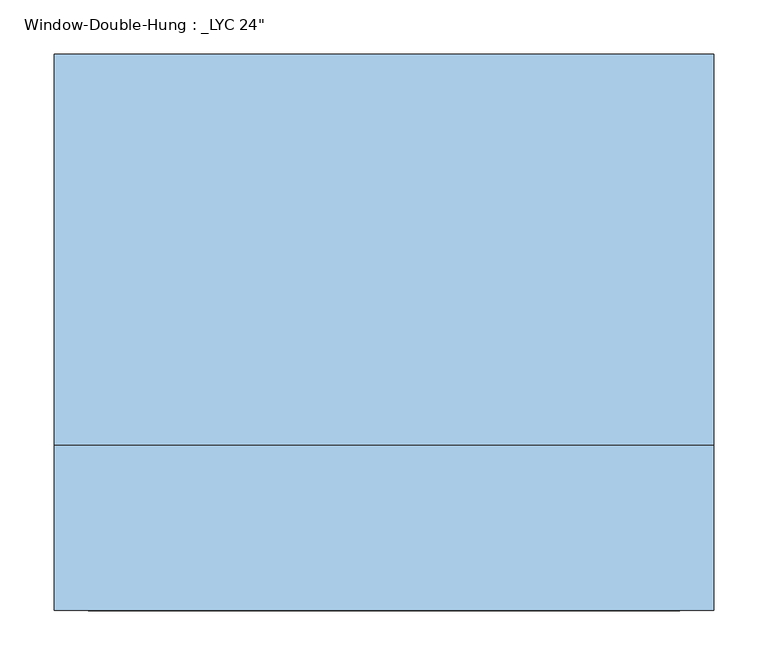
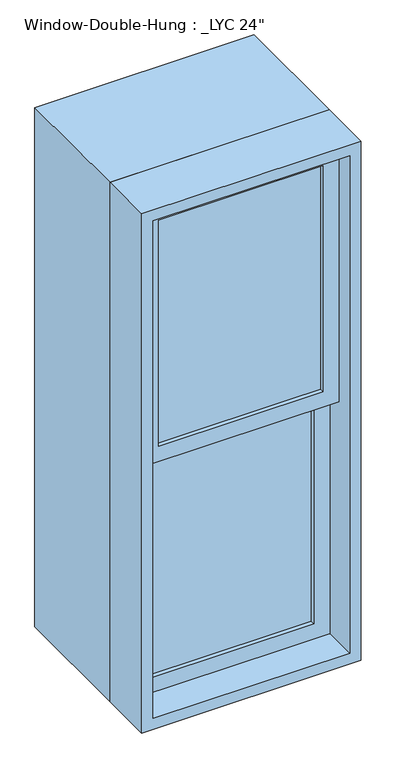
"""IFC4 building model written with IfcOpenShell, lengths in millimetres: window geometry."""

import ifcopenshell
import ifcopenshell.guid

model = None  # the IFC model being written
_history = None  # IfcOwnerHistory: only IFC2X3 demands one
_inside = {}  # id of a spatial element -> (the spatial element, [elements in it])
_under = {}  # id of a project, library or spatial element -> (it, [spatial elements below it])
_declared = {}  # id of a project -> (the project, [libraries it declares])
_typed = {}  # id of a type object -> (the type object, [elements of that type])
_made_of = {}  # id of a material, layer set ... -> (it, [elements and type objects made of it])


def new_model(schema):
    """Start an empty IFC model of exactly this schema.

    Asked for "IFC4X3", IfcOpenShell would pick the latest addendum, in which some entities
    have other attributes; the version numbers below select the first issue.
    IFC2X3 requires an IfcOwnerHistory on every rooted entity: one is made here for all.
    """
    global model, _history
    if schema == "IFC4X3":
        model = ifcopenshell.file(schema_version=(4, 3, 0, 0))
    else:
        model = ifcopenshell.file(schema=schema)
    _inside.clear()
    _under.clear()
    _declared.clear()
    _typed.clear()
    _made_of.clear()
    _history = None
    if model.schema == "IFC2X3":
        org = make("IfcOrganization", Name="unknown")
        user = make(
            "IfcPersonAndOrganization",
            ThePerson=make("IfcPerson", FamilyName="unknown"),
            TheOrganization=org,
        )
        app = make(
            "IfcApplication",
            ApplicationDeveloper=org,
            Version="unknown",
            ApplicationFullName="unknown",
            ApplicationIdentifier="unknown",
        )
        _history = make(
            "IfcOwnerHistory",
            OwningUser=user,
            OwningApplication=app,
            ChangeAction="ADDED",
            CreationDate=0,
        )
    return model


def make(cls, **values):
    """One entity of the class cls with the attributes given. An attribute that is None is left unset."""
    return model.create_entity(
        cls, **{name: value for name, value in values.items() if value is not None}
    )


def rooted(cls, **values):
    """An entity with a GlobalId (a new one), such as an element, a storey or a relation."""
    return make(cls, GlobalId=ifcopenshell.guid.new(), OwnerHistory=_history, **values)


def si_unit(unit_type, name, prefix=None):
    """IfcSIUnit, for example si_unit("LENGTHUNIT", "METRE", prefix="MILLI")."""
    return make("IfcSIUnit", UnitType=unit_type, Prefix=prefix, Name=name)


def assignment(units):
    """IfcUnitAssignment: the units of a project."""
    return None if units is None else make("IfcUnitAssignment", Units=units)


def point(xyz):
    """IfcCartesianPoint."""
    return None if xyz is None else make("IfcCartesianPoint", Coordinates=xyz)


def direction(xyz):
    """IfcDirection."""
    return None if xyz is None else make("IfcDirection", DirectionRatios=xyz)


def frame(location, z_axis=None, x_axis=None):
    """IfcAxis2Placement3D, a coordinate frame: its origin and axes. An axis left out is left unset."""
    return make(
        "IfcAxis2Placement3D",
        Location=point(location),
        Axis=direction(z_axis),
        RefDirection=direction(x_axis),
    )


def origin():
    """The frame at (0, 0, 0) with its axes left unset."""
    return frame((0.0, 0.0, 0.0))


def place(relative_to, where):
    """IfcLocalPlacement: puts the frame where relative to a parent placement (None: the world)."""
    return make(
        "IfcLocalPlacement", PlacementRelTo=relative_to, RelativePlacement=where
    )


def context(
    kind, dimensions, precision=None, world=None, true_north=None, identifier=None
):
    """IfcGeometricRepresentationContext, for example the 3D "Model" context."""
    return make(
        "IfcGeometricRepresentationContext",
        ContextIdentifier=identifier,
        ContextType=kind,
        CoordinateSpaceDimension=dimensions,
        Precision=precision,
        WorldCoordinateSystem=world,
        TrueNorth=true_north,
    )


def project(units=None, contexts=None):
    """IfcProject with its units and contexts."""
    return rooted(
        "IfcProject",
        Name="project",
        RepresentationContexts=contexts,
        UnitsInContext=assignment(units),
    )


def spatial(cls, under=None, at=None, **own):
    """A site, building, storey or space (cls), placed at a placement, below another one or the project."""
    s = rooted(cls, ObjectPlacement=at, **own)
    if under is not None:
        _under.setdefault(under.id(), (under, []))[1].append(s)
    return s


def polyline(points):
    """IfcPolyline through the points."""
    return make("IfcPolyline", Points=[point(p) for p in points])


def outline(outer, holes=None, kind="AREA"):
    """IfcArbitraryClosedProfileDef: a profile drawn as a closed curve; with holes, ...WithVoids."""
    if holes is None:
        return make("IfcArbitraryClosedProfileDef", ProfileType=kind, OuterCurve=outer)
    return make(
        "IfcArbitraryProfileDefWithVoids",
        ProfileType=kind,
        OuterCurve=outer,
        InnerCurves=holes,
    )


def extrude(swept, where, along, depth):
    """IfcExtrudedAreaSolid: the profile swept, set in the frame where, extruded along a direction by depth."""
    return make(
        "IfcExtrudedAreaSolid",
        SweptArea=swept,
        Position=where,
        ExtrudedDirection=direction(along),
        Depth=depth,
    )


def shape(context_of_items, identifier, shape_type, items):
    """IfcShapeRepresentation: the items that make up one representation, for example the "Body"."""
    return make(
        "IfcShapeRepresentation",
        ContextOfItems=context_of_items,
        RepresentationIdentifier=identifier,
        RepresentationType=shape_type,
        Items=items,
    )


def source(mapping_origin, context_of_items, identifier, shape_type, items):
    """IfcRepresentationMap: a shape defined once, which mapped items show again and again."""
    return make(
        "IfcRepresentationMap",
        MappingOrigin=mapping_origin,
        MappedRepresentation=shape(context_of_items, identifier, shape_type, items),
    )


def transform(
    local_origin,
    x_axis=None,
    y_axis=None,
    z_axis=None,
    scale=None,
    scale2=None,
    scale3=None,
    uniform=True,
):
    """IfcCartesianTransformationOperator3D, or its non-uniform kind. x_axis, y_axis, z_axis: its Axis1, 2, 3."""
    if uniform:
        return make(
            "IfcCartesianTransformationOperator3D",
            Axis1=direction(x_axis),
            Axis2=direction(y_axis),
            LocalOrigin=point(local_origin),
            Scale=scale,
            Axis3=direction(z_axis),
        )
    return make(
        "IfcCartesianTransformationOperator3DnonUniform",
        Axis1=direction(x_axis),
        Axis2=direction(y_axis),
        LocalOrigin=point(local_origin),
        Scale=scale,
        Axis3=direction(z_axis),
        Scale2=scale2,
        Scale3=scale3,
    )


def mapped(mapping_source, mapping_target):
    """IfcMappedItem: shows the shape of a source again, moved by a transform."""
    return make(
        "IfcMappedItem", MappingSource=mapping_source, MappingTarget=mapping_target
    )


def made_of(thing, what):
    """Note that an element or type object is made of a material, layer set ...; save() writes the relation."""
    if what is not None:
        _made_of.setdefault(what.id(), (what, []))[1].append(thing)
    return thing


def element(
    cls,
    number,
    at=None,
    inside=None,
    cuts=None,
    type_object=None,
    material=None,
    context=None,
    identifier="Body",
    shape_type=None,
    held_by="IfcProductDefinitionShape",
    body=None,
    shapes=None,
    **own,
):
    """One element of the class cls, such as IfcWall. Its Tag is "e" and its number.

    at: its placement. inside: the storey or other place that contains it. cuts: it is an
    opening in that element (IfcRelVoidsElement). A single representation is given by context,
    identifier, shape_type and body (its items); several are given by shapes. held_by: the class
    of the entity that holds the representations. save() writes the other relations.
    """
    e = rooted(cls, Tag="e%d" % number, ObjectPlacement=at, **own)
    if body is not None:
        shapes = [shape(context, identifier, shape_type, body)]
    if shapes is not None:
        e.Representation = make(held_by, Representations=shapes)
    if inside is not None:
        _inside.setdefault(inside.id(), (inside, []))[1].append(e)
    if cuts is not None:
        rooted(
            "IfcRelVoidsElement", RelatingBuildingElement=cuts, RelatedOpeningElement=e
        )
    if type_object is not None:
        _typed.setdefault(type_object.id(), (type_object, []))[1].append(e)
    return made_of(e, material)


def aggregate(whole, parts):
    """IfcRelAggregates: a whole, such as a stair, and the parts it consists of."""
    return rooted("IfcRelAggregates", RelatingObject=whole, RelatedObjects=parts)


def save(model, path):
    """Write the relations noted so far, then the file.

    IfcRelAggregates (storeys below a building ...), IfcRelContainedInSpatialStructure (elements
    in a storey), IfcRelDefinesByType, IfcRelAssociatesMaterial and IfcRelDeclares: one each for
    every whole, place, type object, material and project.
    """
    for whole, parts in _under.values():
        aggregate(whole, parts)
    for where, things in _inside.values():
        rooted(
            "IfcRelContainedInSpatialStructure",
            RelatedElements=things,
            RelatingStructure=where,
        )
    for kind, things in _typed.values():
        rooted("IfcRelDefinesByType", RelatedObjects=things, RelatingType=kind)
    for what, things in _made_of.values():
        rooted("IfcRelAssociatesMaterial", RelatedObjects=things, RelatingMaterial=what)
    for by, libraries in _declared.values():
        rooted("IfcRelDeclares", RelatingContext=by, RelatedDefinitions=libraries)
    model.write(path)


def window_0b2b9546(model_context):
    return source(origin(), model_context, "Body", "SweptSolid", [
        extrude(outline(polyline([(228.6, -158.75), (-228.6, -158.75), (-228.6, -152.4), (228.6, -152.4), (228.6, -158.75)])), frame((0.0, 0.0, 990.6), z_axis=(0.0, 0.0, 1.0), x_axis=(1.0, 0.0, 0.0)), (0.0, 0.0, 1.0), 663.575),
        extrude(outline(polyline([(-228.6, -146.05), (-228.6, -139.7), (228.6, -139.7), (228.6, -146.05), (-228.6, -146.05)])), frame((0.0, 0.0, 990.6), z_axis=(0.0, 0.0, 1.0), x_axis=(1.0, 0.0, 0.0)), (0.0, 0.0, 1.0), 663.575),
        extrude(outline(polyline([(228.6, -203.2), (-228.6, -203.2), (-228.6, -196.85), (228.6, -196.85), (228.6, -203.2)])), frame((0.0, 0.0, 1698.625), z_axis=(0.0, 0.0, 1.0), x_axis=(1.0, 0.0, 0.0)), (0.0, 0.0, 1.0), 663.575),
        extrude(outline(polyline([(-228.6, -190.5), (-228.6, -184.15), (228.6, -184.15), (228.6, -190.5), (-228.6, -190.5)])), frame((0.0, 0.0, 1698.625), z_axis=(0.0, 0.0, 1.0), x_axis=(1.0, 0.0, 0.0)), (0.0, 0.0, 1.0), 663.575),
        extrude(outline(polyline([(1698.625, 273.05), (1698.625, -273.05), (946.15, -273.05), (946.15, 273.05), (1698.625, 273.05)]), holes=[polyline([(1654.175, -228.6), (1654.175, 228.6), (990.6, 228.6), (990.6, -228.6), (1654.175, -228.6)])]), frame((0.0, -171.45, 0.0), z_axis=(0.0, 1.0, 0.0), x_axis=(0.0, 0.0, 1.0)), (0.0, 0.0, 1.0), 44.45),
        extrude(outline(polyline([(2406.65, 273.05), (2406.65, -273.05), (1654.175, -273.05), (1654.175, 273.05), (2406.65, 273.05)]), holes=[polyline([(2362.2, -228.6), (2362.2, 228.6), (1698.625, 228.6), (1698.625, -228.6), (2362.2, -228.6)])]), frame((0.0, -215.9, 0.0), z_axis=(0.0, 1.0, 0.0), x_axis=(0.0, 0.0, 1.0)), (0.0, 0.0, 1.0), 44.45),
        extrude(outline(polyline([(2438.4, 304.8), (2438.4, -304.8), (914.4, -304.8), (914.4, 304.8), (2438.4, 304.8)]), holes=[polyline([(2406.65, -273.05), (2406.65, 273.05), (946.15, 273.05), (946.15, -273.05), (2406.65, -273.05)])]), frame((0.0, -266.7, 0.0), z_axis=(0.0, 1.0, 0.0), x_axis=(0.0, 0.0, 1.0)), (0.0, 0.0, 1.0), 152.4),
        extrude(outline(polyline([(2438.4, 304.8), (2438.4, -304.8), (914.4, -304.8), (914.4, 304.8), (2438.4, 304.8)]), holes=[polyline([(2419.35, 285.75), (933.45, 285.75), (933.45, -285.75), (2419.35, -285.75), (2419.35, 285.75)])]), frame((0.0, -114.3, 0.0), z_axis=(0.0, 1.0, 0.0), x_axis=(0.0, 0.0, 1.0)), (0.0, 0.0, 1.0), 361.95),
    ])


if __name__ == "__main__":
    model = new_model("IFC4")
    model_context = context("Model", 3, world=origin())
    ifc_project = project(units=[si_unit("LENGTHUNIT", "METRE", prefix="MILLI")], contexts=[model_context])
    site = spatial("IfcSite", under=ifc_project)
    building = spatial("IfcBuilding", under=site)
    placement = place(None, origin())
    window_shape = window_0b2b9546(model_context)
    element("IfcWindow", 1, ObjectType="Window-Double-Hung : _LYC 24\"", at=placement, inside=building, context=model_context, shape_type="MappedRepresentation", body=[
        mapped(window_shape, transform((0.0, 0.0, 0.0), x_axis=(1.0, 0.0, 0.0), y_axis=(0.0, 1.0, 0.0), z_axis=(0.0, 0.0, 1.0))),
    ])
    save(model, "model.ifc")

# Revit data of these elements
# Type "Window-Double-Hung : _LYC 24\""
#   Type Mark = "23"
#   Fire Rating = "0.5h"
#   Assembly Code = "B2020100"
#   Wall Thickness [instance default] = 0' - 6"
#   Visual Light Transmittance = 0.9
#   Thermal Resistance (R) = 1.8146 (h·ft²·°F)/BTU
#   Solar Heat Gain Coefficient = 0.78
#   Rough Width = 2' - 0 1/2"
#   Rough Height = 5' - 0 1/2"
#   Muntin Width = 1' - 6"
#   Muntin Height = 2' - 2 1/8"
#   Interior Wall Closure [instance default] = 0' - 1 1/2"
#   Heat Transfer Coefficient (U) = 0.6496 BTU/(h·ft²·°F)
#   Frame Extension [instance default] = 0' - 2"
#   Exterior Wall Closure [instance default] = 0' - 0 1/2"
#   Extension Jamb [instance default] = 0' - 0 3/4"
#   Height = 5' - 0"
#   Width = 2' - 0"
#   Window Inset [instance default] = 0' - 0 3/4"
#   Top Muntin Visibility = yes
#   Interior Trim Visibility [instance default] = yes
#   Indicator Visibility [instance default] = yes
#   Exterior Trim Visibility [instance default] = yes
#   Extension Jamb Visibility [instance default] = yes
#   Define Thermal Properties by = 1
#   Bottom Muntin Visibility = yes
#   Muntin Pattern = Muntin Pattern_2x2 : Muntin Pattern_2x2
#   Interior Trim Material = Wood - Stained
#   Interior Trim = Trim-Window-Interior-Flat : Picture Frame
#   Interior Frame Material = Wood - Stained
#   Glass Panel Material = Glass
#   Exterior Trim Material = Clad - White
#   Exterior Trim = Trim-Window-Exterior-Flat : with Sill
#   Exterior Frame Material = Clad - White
#   Construction Type Id = ""
#   Wall Closure = (empty or 0)
#   Analytic Construction = (empty or 0)
# Element 1 (IfcWindow, "Window-Double-Hung : _LYC 24\"")
#   Wall Thickness = 1' - 7 1/2"
#   Extension Jamb = 1' - 2 1/4"
#   Materials on its faces: "Wood - Stained", "Glass", "Clad - White"
# Materials
#   "Wood - Stained": class "Wood", colour RGB 224 178 126, transparency 0, Cost = 0
#   "Glass": class "Unassigned", colour RGB 0 128 192, transparency 0.75
#   "Clad - White": class "Wood", colour RGB 242 242 238, transparency 0, Cost = 0
